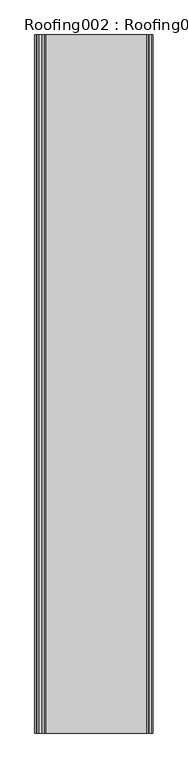
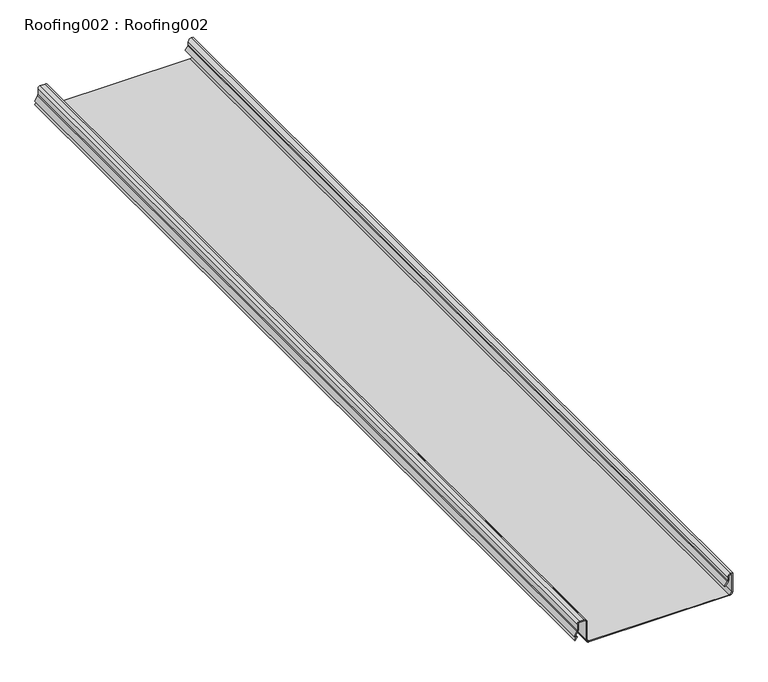
"""IFC4 building model written with IfcOpenShell, lengths in millimetres: proxy geometry, Roofing002 : Roofing002."""

from ifc_helpers import new_model, si_unit, point, frame, frame_2d, origin, place, context, project, spatial, polyline, circle_curve, trimmed, segment, composite_curve, outline, extrude, source, transform, mapped, element, save


def roofing002_roofing002_2d5ec91b(model_context):
    return source(origin(), model_context, "Body", "SweptSolid", [
        extrude(outline(composite_curve([segment(trimmed(circle_curve(frame_2d((43490.7540667, -5199.4144727)), 5.08), [point((43487.7710372, -5195.3025467))], [point((43490.7540667, -5194.3344727))], False, "CARTESIAN"), True, "CONTINUOUS"), segment(polyline([(43490.7540667, -5194.3344727), (43497.510625, -5194.3344727)]), True, "CONTINUOUS"), segment(trimmed(circle_curve(frame_2d((43497.510625, -5189.2544727)), 5.08), [point((43497.510625, -5194.3344727))], [point((43502.590625, -5189.2544727))], True, "CARTESIAN"), True, "CONTINUOUS"), segment(polyline([(43502.590625, -5189.2544727), (43502.590625, -5187.659668), (43462.8534375, -5187.659668)]), True, "CONTINUOUS"), segment(trimmed(circle_curve(frame_2d((43462.8534375, -5192.739668)), 5.08), [point((43462.8534375, -5187.659668))], [point((43457.7734375, -5192.739668))], True, "CARTESIAN"), True, "CONTINUOUS"), segment(polyline([(43457.7734375, -5192.739668), (43457.7734375, -5493.01375)]), True, "CONTINUOUS"), segment(trimmed(circle_curve(frame_2d((43462.8534375, -5493.01375)), 5.08), [point((43457.7734375, -5493.01375))], [point((43462.8534375, -5498.09375))], True, "CARTESIAN"), True, "CONTINUOUS"), segment(polyline([(43462.8534375, -5498.09375), (43504.466875, -5498.09375)]), True, "CONTINUOUS"), segment(trimmed(circle_curve(frame_2d((43504.466875, -5503.17375)), 5.08), [point((43504.466875, -5498.09375))], [point((43509.546875, -5503.17375))], False, "CARTESIAN"), True, "CONTINUOUS"), segment(polyline([(43509.546875, -5503.17375), (43509.546875, -5513.1815269)]), True, "CONTINUOUS"), segment(trimmed(circle_curve(frame_2d((43504.466875, -5513.1815269)), 5.08), [point((43509.546875, -5513.1815269))], [point((43504.466875, -5518.2615269))], False, "CARTESIAN"), True, "CONTINUOUS"), segment(polyline([(43504.466875, -5518.2615269), (43491.2843008, -5518.2615269)]), True, "CONTINUOUS"), segment(trimmed(circle_curve(frame_2d((43491.2843008, -5523.3415269)), 5.08), [point((43491.2843008, -5518.2615269))], [point((43488.7802894, -5518.9215352))], True, "CARTESIAN"), True, "CONTINUOUS"), segment(polyline([(43488.7802894, -5518.9215352), (43478.2226563, -5524.9026402), (43475.78125, -5520.7385777), (43470.1796875, -5524.7376011), (43469.0176138, -5523.1098466), (43476.399929, -5517.8395222), (43478.9513272, -5522.191187), (43487.7944581, -5517.181381)]), True, "CONTINUOUS"), segment(trimmed(circle_curve(frame_2d((43491.2843008, -5523.3415269)), 7.08), [point((43487.7944581, -5517.181381))], [point((43491.2843008, -5516.2615269))], False, "CARTESIAN"), True, "CONTINUOUS"), segment(polyline([(43491.2843008, -5516.2615269), (43504.466875, -5516.2615269)]), True, "CONTINUOUS"), segment(trimmed(circle_curve(frame_2d((43504.466875, -5513.1815269)), 3.08), [point((43504.466875, -5516.2615269))], [point((43507.546875, -5513.1815269))], True, "CARTESIAN"), True, "CONTINUOUS"), segment(polyline([(43507.546875, -5513.1815269), (43507.546875, -5503.17375)]), True, "CONTINUOUS"), segment(trimmed(circle_curve(frame_2d((43504.466875, -5503.17375)), 3.08), [point((43507.546875, -5503.17375))], [point((43504.466875, -5500.09375))], True, "CARTESIAN"), True, "CONTINUOUS"), segment(polyline([(43504.466875, -5500.09375), (43462.8534375, -5500.09375)]), True, "CONTINUOUS"), segment(trimmed(circle_curve(frame_2d((43462.8534375, -5493.01375)), 7.08), [point((43462.8534375, -5500.09375))], [point((43455.7734375, -5493.01375))], False, "CARTESIAN"), True, "CONTINUOUS"), segment(polyline([(43455.7734375, -5493.01375), (43455.7734375, -5192.739668)]), True, "CONTINUOUS"), segment(trimmed(circle_curve(frame_2d((43462.8534375, -5192.739668)), 7.08), [point((43455.7734375, -5192.739668))], [point((43462.8534375, -5185.659668))], False, "CARTESIAN"), True, "CONTINUOUS"), segment(polyline([(43462.8534375, -5185.659668), (43504.590625, -5185.659668), (43504.590625, -5189.2544727)]), True, "CONTINUOUS"), segment(trimmed(circle_curve(frame_2d((43497.510625, -5189.2544727)), 7.08), [point((43504.590625, -5189.2544727))], [point((43497.510625, -5196.3344727))], False, "CARTESIAN"), True, "CONTINUOUS"), segment(polyline([(43497.510625, -5196.3344727), (43490.7540667, -5196.3344727)]), True, "CONTINUOUS"), segment(trimmed(circle_curve(frame_2d((43490.7540667, -5199.4144727)), 3.08), [point((43490.7540667, -5196.3344727))], [point((43488.9454582, -5196.9214152))], True, "CARTESIAN"), True, "CONTINUOUS"), segment(polyline([(43488.9454582, -5196.9214152), (43480.4712961, -5203.0690638), (43479.296875, -5201.4501953), (43487.7710372, -5195.3025467)]), True, "CONTINUOUS")], self_intersect=False)), frame((0.0, 7982.1531721, 0.0), z_axis=(0.0, 1.0, 0.0), x_axis=(0.0, 0.0, 1.0)), (0.0, 0.0, 1.0), 2000.0),
    ])


if __name__ == "__main__":
    model = new_model("IFC4")
    model_context = context("Model", 3, world=origin())
    ifc_project = project(units=[si_unit("LENGTHUNIT", "METRE", prefix="MILLI")], contexts=[model_context])
    site = spatial("IfcSite", under=ifc_project)
    building = spatial("IfcBuilding", under=site)
    placement = place(None, origin())
    roofing002_roofing002_shape = roofing002_roofing002_2d5ec91b(model_context)
    element("IfcBuildingElementProxy", 1, Name="Roofing002 : Roofing002", ObjectType="Roofing002 : Roofing002", at=placement, inside=building, context=model_context, shape_type="MappedRepresentation", body=[
        mapped(roofing002_roofing002_shape, transform((0.0, 0.0, 0.0), x_axis=(1.0, 0.0, 0.0), y_axis=(0.0, 1.0, 0.0), z_axis=(0.0, 0.0, 1.0))),
    ])
    save(model, "model.ifc")

# Revit data of these elements
# Type "Roofing002 : Roofing002"
#   NameOverride = "Roofing002"
# Element 1 (IfcBuildingElementProxy, "Roofing002 : Roofing002")
#   Materials on its faces: "STANDING SEAM METAL ROOF"
# Materials
#   "STANDING SEAM METAL ROOF": class "Unassigned", colour RGB 128 128 128, transparency 0
